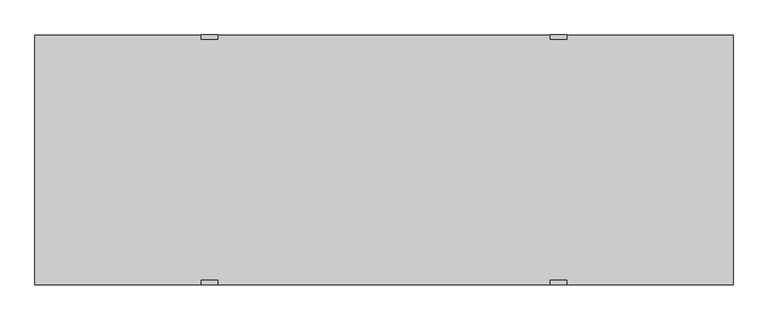
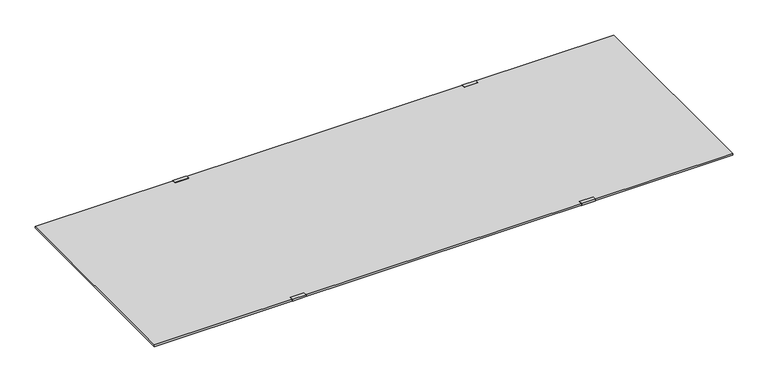
"""IFC4 building model written with IfcOpenShell, lengths in millimetres: proxy geometry."""

from ifc_helpers import new_model, si_unit, frame, origin, origin_with_axes, place, context, project, spatial, polyline, outline, extrude, source, transform, mapped, element, save


def specialty_equipment_ebe82977(model_context):
    return source(origin(), model_context, "Body", "SweptSolid", [
        extrude(outline(polyline([(381.0, 6.35), (368.3, 6.35), (368.3, 7.14375), (381.79375, 7.14375), (381.79375, 0.0), (381.0, 0.0), (381.0, 6.35)])), frame((508.0, 0.0, 0.0), z_axis=(1.0, 0.0, 0.0), x_axis=(0.0, 1.0, 0.0)), (0.0, 0.0, 1.0), 50.8),
        extrude(outline(polyline([(381.0, 6.35), (368.3, 6.35), (368.3, 7.14375), (381.79375, 7.14375), (381.79375, 0.0), (381.0, 0.0), (381.0, 6.35)])), frame((-558.8, 0.0, 0.0), z_axis=(1.0, 0.0, 0.0), x_axis=(0.0, 1.0, 0.0)), (0.0, 0.0, 1.0), 50.8),
        extrude(outline(polyline([(-381.0, 6.35), (-381.0, 0.0), (-381.79375, 0.0), (-381.79375, 7.14375), (-368.3, 7.14375), (-368.3, 6.35), (-381.0, 6.35)])), frame((508.0, 0.0, 0.0), z_axis=(1.0, 0.0, 0.0), x_axis=(0.0, 1.0, 0.0)), (0.0, 0.0, 1.0), 50.8),
        extrude(outline(polyline([(-381.0, 6.35), (-381.0, 0.0), (-381.79375, 0.0), (-381.79375, 7.14375), (-368.3, 7.14375), (-368.3, 6.35), (-381.0, 6.35)])), frame((-558.8, 0.0, 0.0), z_axis=(1.0, 0.0, 0.0), x_axis=(0.0, 1.0, 0.0)), (0.0, 0.0, 1.0), 50.8),
        extrude(outline(polyline([(1066.8, -381.0), (-1066.8, -381.0), (-1066.8, 381.0), (1066.8, 381.0), (1066.8, -381.0)])), origin_with_axes(), (0.0, 0.0, 1.0), 6.35),
    ])


if __name__ == "__main__":
    model = new_model("IFC4")
    model_context = context("Model", 3, world=origin())
    ifc_project = project(units=[si_unit("LENGTHUNIT", "METRE", prefix="MILLI")], contexts=[model_context])
    site = spatial("IfcSite", under=ifc_project)
    building = spatial("IfcBuilding", under=site)
    placement = place(None, origin())
    specialty_equipment_shape = specialty_equipment_ebe82977(model_context)
    element("IfcBuildingElementProxy", 1, Name="Bradley-Washroom_Accessories-Mirrors-747_Standard : 84\" x 36\" + BradEX", ObjectType="Bradley-Washroom_Accessories-Mirrors-747_Standard : 84\" x 36\" + BradEX", at=placement, inside=building, context=model_context, shape_type="MappedRepresentation", body=[
        mapped(specialty_equipment_shape, transform((0.0, 0.0, 0.0), x_axis=(1.0, 0.0, 0.0), y_axis=(0.0, 1.0, 0.0), z_axis=(0.0, 0.0, 1.0))),
    ])
    save(model, "model.ifc")

# Revit data of these elements
# Type "Bradley-Washroom_Accessories-Mirrors-747_Standard : 84\" x 36\" + BradEX"
#   Keynote = "M08831300.01"
#   Warranty Information = "Complete unit, excepting mirrors warranted for one year.\r\n Stainless steel mirror frames for fifteen years.\r\n Plate glass mirrors for fifteen years.\r\n This warranty does not cover installation or any other labor charges and does not apply to any units,\r\n which have been damaged by accident, abuse, improper installation, improper maintenance, or altered in any way."
#   Version = "1.0"
#   URL = "http://www.bradleycorp.com/"
#   Type Comments = "BradEX 1/4\" Float Glass Mirror"
#   OmniClass Title = "Mirrors"
#   OmniClass Code = "23.40.95.17.17"
#   Modeling Code = ""
#   Model = "747-024360"
#   MasterFormat Title = "Commercial Toilet Accessories"
#   MasterFormat Number = "10 28 13. 13"
#   Manufacturer = "Bradley Corporation"
#   Industry Standards = "ASTM C 1036"
#   Fire Rating = "n/a"
#   Description = "Frameless Mirror, Clip Fasteners, 24 by 36 inches"
#   Copyright = "This Model Data is Property of Bradley Corporation"
#   Buy American Act = "Yes"
#   Assembly Code = "C1030900"
#   ADA Compliant = "Yes"
#   Width = 7' - 0"
#   Height = 2' - 6"
#   Fastener Placement = 1' - 9"
#   Depth = 0' - 0 1/4"
#   Default Elevation = 3' - 4"
#   Reflective Material = Glass - Bradley Corp - BradEX - Polished Float Mirror
#   Frame Material = Bradley Corp Stainless Steel - Satin
# Element 1 (IfcBuildingElementProxy, "Bradley-Washroom_Accessories-Mirrors-747_Standard : 84\" x 36\" + BradEX")
#   Materials on its faces: "Bradley Corp Stainless Steel - Satin", "Glass - Bradley Corp - BradEX - Polished Float Mirror"
# Materials
#   "Glass - Bradley Corp - BradEX - Polished Float Mirror": class "Glass", colour RGB 220 232 220, transparency 0, Manufacturer = "Bradley Corporation", URL = "www.bradleycorp.com", Description = "Stainless Steel - Satin Finish", Cost = 0
#   "Bradley Corp Stainless Steel - Satin": class "Metal", colour RGB 189 187 185, transparency 0, Manufacturer = "Bradley Corporation", URL = "www.bradleycorp.com", Description = "Stainless Steel - Satin Finish", Cost = 0
